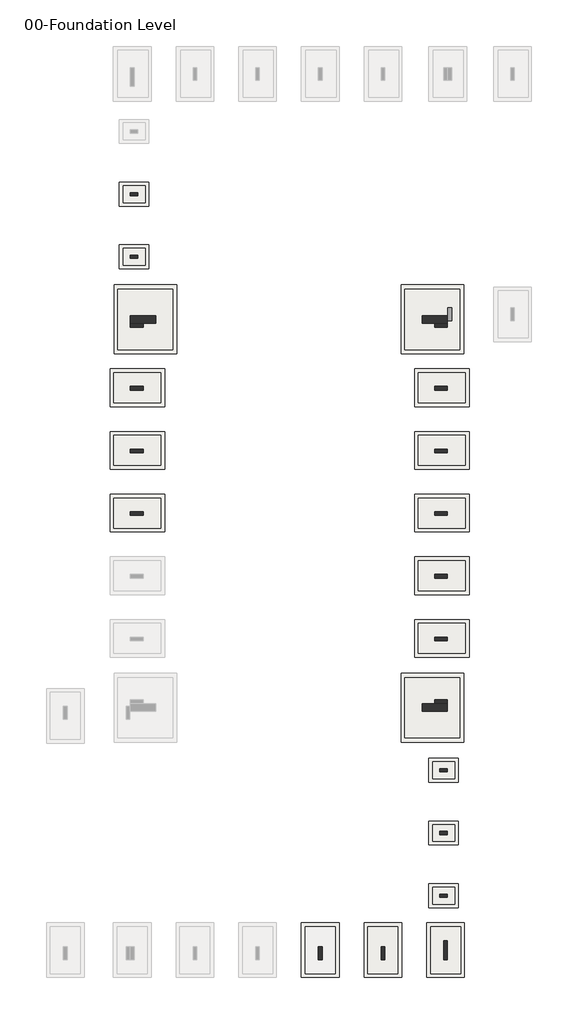
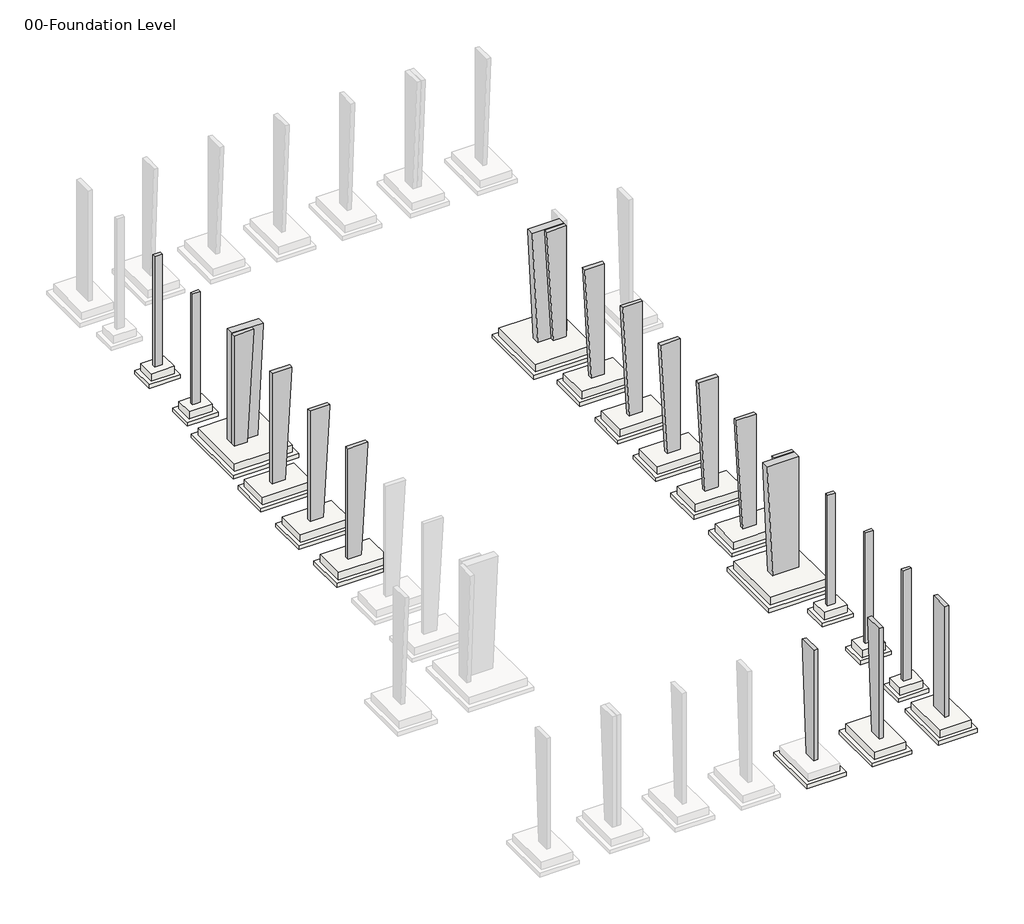
# One storey, part 2 of 4: 37 slabs, 22 columns.
"""IFC4 building model written with IfcOpenShell, lengths in millimetres."""

from ifc_helpers import new_model, si_unit, frame, origin, place, context, project, spatial, polyline, outline, extrude, faceted_brep, element, save

model = new_model("IFC4")

# Units and contexts
model_context = context("Model", 3, world=origin())
ifc_project = project(units=[si_unit("LENGTHUNIT", "METRE", prefix="MILLI")], contexts=[model_context])

# Site, building, storey
site = spatial("IfcSite", under=ifc_project)
building = spatial("IfcBuilding", under=site)
storey = spatial("IfcBuildingStorey", under=building, Name="00-Foundation Level", Elevation=-2000.0)

# Columns
placement = place(None, origin())
element("IfcColumn", 1, ObjectType="Frame Col.2 : 1500x300", at=placement, inside=storey, context=model_context, shape_type="Brep", body=[
    faceted_brep([(49483.2245514, 20339.9999998, -1100.0), (50483.2245514, 20339.9999998, -1100.0), (50483.2245514, 20339.9999998, 7800.0), (48983.2245514, 20339.9999998, 7800.0), (48989.9661245, 20339.9999998, 7680.0), (48983.2245514, 20639.9999998, 7800.0), (48989.9661245, 20639.9999998, 7680.0), (49483.2245514, 20639.9999998, -1100.0), (50483.2245514, 20639.9999998, -1100.0), (50483.2245514, 20639.9999998, 7800.0), (50483.2245514, 20639.9999998, 7680.0)], [[[0, 1, 2, 3, 4]], [[0, 4, 3, 5, 6, 7]], [[8, 7, 6, 5, 9, 10]], [[2, 1, 8, 10, 9]], [[1, 0, 7, 8]], [[3, 2, 9, 5]]]),
])
element("IfcColumn", 2, ObjectType="Frame Col.2 : 1500x300", at=placement, inside=storey, context=model_context, shape_type="Brep", body=[
    faceted_brep([(40183.2245515, 899.7448196, -1100.0), (40183.2245515, -100.2551804, -1100.0), (40183.2245515, -100.2551804, 7680.0), (40183.2245515, -100.2551804, 7800.0), (40183.2245515, 1399.7448196, 7800.0), (40183.2245515, 1393.0032466, 7680.0), (40483.2245515, 1399.7448196, 7800.0), (40483.2245515, 1393.0032466, 7680.0), (40483.2245515, 899.7448196, -1100.0), (40483.2245515, -100.2551804, -1100.0), (40483.2245515, -100.2551804, 7800.0), (40483.2245515, -100.2551804, 7680.0)], [[[0, 1, 2, 3, 4, 5]], [[0, 5, 4, 6, 7, 8]], [[9, 8, 7, 6, 10, 11]], [[3, 2, 1, 9, 11, 10]], [[1, 0, 8, 9]], [[4, 3, 10, 6]]]),
])
element("IfcColumn", 3, ObjectType="Frame Col.2 : 1500x300", at=placement, inside=storey, context=model_context, shape_type="Brep", body=[
    faceted_brep([(45183.2245515, 899.7448196, -1100.0), (45183.2245515, -100.2551804, -1100.0), (45183.2245515, -100.2551804, 7680.0), (45183.2245515, -100.2551804, 7800.0), (45183.2245515, 1399.7448196, 7800.0), (45183.2245515, 1393.0032466, 7680.0), (45483.2245515, 1399.7448196, 7800.0), (45483.2245515, 1393.0032466, 7680.0), (45483.2245515, 899.7448196, -1100.0), (45483.2245515, -100.2551804, -1100.0), (45483.2245515, -100.2551804, 7800.0), (45483.2245515, -100.2551804, 7680.0)], [[[0, 1, 2, 3, 4, 5]], [[0, 5, 4, 6, 7, 8]], [[9, 8, 7, 6, 10, 11]], [[3, 2, 1, 9, 11, 10]], [[1, 0, 8, 9]], [[4, 3, 10, 6]]]),
])
element("IfcColumn", 4, ObjectType="Frame Col.2 : 1500x300", at=placement, inside=storey, context=model_context, shape_type="Brep", body=[
    faceted_brep([(49483.2245514, 25339.9999988, -1100.0), (50483.2245514, 25339.9999988, -1100.0), (50483.2245514, 25339.9999988, 7680.0), (50483.2245514, 25339.9999988, 7800.0), (48983.2245514, 25339.9999988, 7800.0), (48989.9661245, 25339.9999988, 7680.0), (49067.4942144, 25339.9999988, 6300.0), (48983.2245514, 25639.9999988, 7800.0), (48989.9661245, 25639.9999988, 7680.0), (49067.4942144, 25639.9999988, 6300.0), (49483.2245514, 25639.9999988, -1100.0), (50483.2245514, 25639.9999988, -1100.0), (50483.2245514, 25639.9999988, 7800.0), (50483.2245514, 25639.9999988, 7680.0)], [[[0, 1, 2, 3, 4, 5, 6]], [[0, 6, 5, 4, 7, 8, 9, 10]], [[11, 10, 9, 8, 7, 12, 13]], [[3, 2, 1, 11, 13, 12]], [[1, 0, 10, 11]], [[4, 3, 12, 7]]]),
])
element("IfcColumn", 5, ObjectType="Frame Col.2 : 1500x300", at=placement, inside=storey, context=model_context, shape_type="Brep", body=[
    faceted_brep([(49483.2245514, 30339.9999988, -1100.0), (50483.2245514, 30339.9999988, -1100.0), (50483.2245514, 30339.9999988, 7680.0), (50483.2245514, 30339.9999988, 7800.0), (48983.2245514, 30339.9999988, 7800.0), (48989.9661245, 30339.9999988, 7680.0), (49067.4942144, 30339.9999988, 6300.0), (48983.2245514, 30639.9999988, 7800.0), (48989.9661245, 30639.9999988, 7680.0), (49067.4942144, 30639.9999988, 6300.0), (49483.2245514, 30639.9999988, -1100.0), (50483.2245514, 30639.9999988, -1100.0), (50483.2245514, 30639.9999988, 7800.0), (50483.2245514, 30639.9999988, 7680.0)], [[[0, 1, 2, 3, 4, 5, 6]], [[0, 6, 5, 4, 7, 8, 9, 10]], [[11, 10, 9, 8, 7, 12, 13]], [[3, 2, 1, 11, 13, 12]], [[1, 0, 10, 11]], [[4, 3, 12, 7]]]),
])
element("IfcColumn", 6, ObjectType="Frame Col.2 : 1500x300", at=placement, inside=storey, context=model_context, shape_type="Brep", body=[
    faceted_brep([(49483.2245514, 35339.9999988, -1100.0), (50483.2245514, 35339.9999988, -1100.0), (50483.2245514, 35339.9999988, 7680.0), (50483.2245514, 35339.9999988, 7800.0), (48983.2245514, 35339.9999988, 7800.0), (48989.9661245, 35339.9999988, 7680.0), (49067.4942144, 35339.9999988, 6300.0), (48983.2245514, 35639.9999988, 7800.0), (48989.9661245, 35639.9999988, 7680.0), (49067.4942144, 35639.9999988, 6300.0), (49483.2245514, 35639.9999988, -1100.0), (50483.2245514, 35639.9999988, -1100.0), (50483.2245514, 35639.9999988, 7800.0), (50483.2245514, 35639.9999988, 7680.0)], [[[0, 1, 2, 3, 4, 5, 6]], [[0, 6, 5, 4, 7, 8, 9, 10]], [[11, 10, 9, 8, 7, 12, 13]], [[3, 2, 1, 11, 13, 12]], [[1, 0, 10, 11]], [[4, 3, 12, 7]]]),
])
element("IfcColumn", 7, ObjectType="Frame Col.2 : 1500x300", at=placement, inside=storey, context=model_context, shape_type="Brep", body=[
    faceted_brep([(26183.2245516, 35639.9999988, -1100.0), (25183.2245516, 35639.9999988, -1100.0), (25183.2245516, 35639.9999988, 7680.0), (25183.2245516, 35639.9999988, 7800.0), (26683.2245516, 35639.9999988, 7800.0), (26676.4829785, 35639.9999988, 7680.0), (26598.9548887, 35639.9999988, 6300.0), (26683.2245516, 35339.9999988, 7800.0), (26676.4829785, 35339.9999988, 7680.0), (26598.9548887, 35339.9999988, 6300.0), (26183.2245516, 35339.9999988, -1100.0), (25183.2245516, 35339.9999988, -1100.0), (25183.2245516, 35339.9999988, 7800.0), (25183.2245516, 35339.9999988, 7680.0)], [[[0, 1, 2, 3, 4, 5, 6]], [[0, 6, 5, 4, 7, 8, 9, 10]], [[11, 10, 9, 8, 7, 12, 13]], [[3, 2, 1, 11, 13, 12]], [[1, 0, 10, 11]], [[4, 3, 12, 7]]]),
])
element("IfcColumn", 8, ObjectType="Frame Col.2 : 1500x300", at=placement, inside=storey, context=model_context, shape_type="Brep", body=[
    faceted_brep([(49483.2245514, 40339.9999988, -1100.0), (50483.2245514, 40339.9999988, -1100.0), (50483.2245514, 40339.9999988, 7680.0), (50483.2245514, 40339.9999988, 7800.0), (48983.2245514, 40339.9999988, 7800.0), (48989.9661245, 40339.9999988, 7680.0), (49067.4942144, 40339.9999988, 6300.0), (48983.2245514, 40639.9999988, 7800.0), (48989.9661245, 40639.9999988, 7680.0), (49067.4942144, 40639.9999988, 6300.0), (49483.2245514, 40639.9999988, -1100.0), (50483.2245514, 40639.9999988, -1100.0), (50483.2245514, 40639.9999988, 7800.0), (50483.2245514, 40639.9999988, 7680.0)], [[[0, 1, 2, 3, 4, 5, 6]], [[0, 6, 5, 4, 7, 8, 9, 10]], [[11, 10, 9, 8, 7, 12, 13]], [[3, 2, 1, 11, 13, 12]], [[1, 0, 10, 11]], [[4, 3, 12, 7]]]),
])
element("IfcColumn", 9, ObjectType="Frame Col.2 : 1500x300", at=placement, inside=storey, context=model_context, shape_type="Brep", body=[
    faceted_brep([(26183.2245516, 40639.9999988, -1100.0), (25183.2245516, 40639.9999988, -1100.0), (25183.2245516, 40639.9999988, 7680.0), (25183.2245516, 40639.9999988, 7800.0), (26683.2245516, 40639.9999988, 7800.0), (26676.4829785, 40639.9999988, 7680.0), (26598.9548887, 40639.9999988, 6300.0), (26683.2245516, 40339.9999988, 7800.0), (26676.4829785, 40339.9999988, 7680.0), (26598.9548887, 40339.9999988, 6300.0), (26183.2245516, 40339.9999988, -1100.0), (25183.2245516, 40339.9999988, -1100.0), (25183.2245516, 40339.9999988, 7800.0), (25183.2245516, 40339.9999988, 7680.0)], [[[0, 1, 2, 3, 4, 5, 6]], [[0, 6, 5, 4, 7, 8, 9, 10]], [[11, 10, 9, 8, 7, 12, 13]], [[3, 2, 1, 11, 13, 12]], [[1, 0, 10, 11]], [[4, 3, 12, 7]]]),
])
element("IfcColumn", 10, ObjectType="Frame Col.2 : 1500x300", at=placement, inside=storey, context=model_context, shape_type="Brep", body=[
    faceted_brep([(49483.2245514, 45339.9999993, -1100.0), (50483.2245514, 45339.9999993, -1100.0), (50483.2245514, 45339.9999993, 7680.0), (50483.2245514, 45339.9999993, 7800.0), (48983.2245514, 45339.9999993, 7800.0), (48989.9661245, 45339.9999993, 7680.0), (49067.4942144, 45339.9999993, 6300.0), (48983.2245514, 45639.9999993, 7800.0), (48989.9661245, 45639.9999993, 7680.0), (49067.4942144, 45639.9999993, 6300.0), (49483.2245514, 45639.9999993, -1100.0), (50483.2245514, 45639.9999993, -1100.0), (50483.2245514, 45639.9999993, 7800.0), (50483.2245514, 45639.9999993, 7680.0)], [[[0, 1, 2, 3, 4, 5, 6]], [[0, 6, 5, 4, 7, 8, 9, 10]], [[11, 10, 9, 8, 7, 12, 13]], [[3, 2, 1, 11, 13, 12]], [[1, 0, 10, 11]], [[4, 3, 12, 7]]]),
])
element("IfcColumn", 11, ObjectType="Frame Col.2 : 1500x300", at=placement, inside=storey, context=model_context, shape_type="Brep", body=[
    faceted_brep([(26183.2245516, 45639.9999993, -1100.0), (25183.2245516, 45639.9999993, -1100.0), (25183.2245516, 45639.9999993, 7680.0), (25183.2245516, 45639.9999993, 7800.0), (26683.2245516, 45639.9999993, 7800.0), (26676.4829785, 45639.9999993, 7680.0), (26598.9548887, 45639.9999993, 6300.0), (26683.2245516, 45339.9999993, 7800.0), (26676.4829785, 45339.9999993, 7680.0), (26598.9548887, 45339.9999993, 6300.0), (26183.2245516, 45339.9999993, -1100.0), (25183.2245516, 45339.9999993, -1100.0), (25183.2245516, 45339.9999993, 7800.0), (25183.2245516, 45339.9999993, 7680.0)], [[[0, 1, 2, 3, 4, 5, 6]], [[0, 6, 5, 4, 7, 8, 9, 10]], [[11, 10, 9, 8, 7, 12, 13]], [[3, 2, 1, 11, 13, 12]], [[1, 0, 10, 11]], [[4, 3, 12, 7]]]),
])
element("IfcColumn", 12, ObjectType="Frame Col.2 : 1500x300", at=placement, inside=storey, context=model_context, shape_type="Brep", body=[
    faceted_brep([(49483.2245514, 50339.9999991, -1100.0), (50483.2245514, 50339.9999991, -1100.0), (50483.2245514, 50339.9999991, 7680.0), (50483.2245514, 50339.9999991, 7800.0), (48983.2245514, 50339.9999991, 7800.0), (48989.9661245, 50339.9999991, 7680.0), (48983.2245514, 50639.9999991, 7800.0), (48989.9661245, 50639.9999991, 7680.0), (49483.2245514, 50639.9999991, -1100.0), (50483.2245514, 50639.9999991, -1100.0), (50483.2245514, 50639.9999991, 7800.0)], [[[0, 1, 2, 3, 4, 5]], [[0, 5, 4, 6, 7, 8]], [[9, 8, 7, 6, 10]], [[3, 2, 1, 9, 10]], [[1, 0, 8, 9]], [[4, 3, 10, 6]]]),
])
element("IfcColumn", 13, ObjectType="Frame Col.2 : 1500x300", at=placement, inside=storey, context=model_context, shape_type="Brep", body=[
    faceted_brep([(26183.2245516, 50639.9999991, -1100.0), (25183.2245516, 50639.9999991, -1100.0), (25183.2245516, 50639.9999991, 7800.0), (26683.2245516, 50639.9999991, 7800.0), (26676.4829785, 50639.9999991, 7680.0), (26683.2245516, 50339.9999991, 7800.0), (26676.4829785, 50339.9999991, 7680.0), (26183.2245516, 50339.9999991, -1100.0), (25183.2245516, 50339.9999991, -1100.0), (25183.2245516, 50339.9999991, 7800.0), (25183.2245516, 50339.9999991, 7680.0)], [[[0, 1, 2, 3, 4]], [[0, 4, 3, 5, 6, 7]], [[8, 7, 6, 5, 9, 10]], [[2, 1, 8, 10, 9]], [[1, 0, 7, 8]], [[3, 2, 9, 5]]]),
])
element("IfcColumn", 14, ObjectType="Frame Col.2 : 2400x600", at=placement, inside=storey, context=model_context, shape_type="Brep", body=[
    faceted_brep([(48483.2245514, 50679.9999988, -1100.0), (50483.2245514, 50679.9999988, -1100.0), (50483.2245514, 50679.9999988, 7800.0), (48083.2245514, 50679.9999988, 7800.0), (48088.6178099, 50679.9999988, 7680.0), (48083.2245514, 51279.9999988, 7800.0), (48088.6178099, 51279.9999988, 7680.0), (48483.2245514, 51279.9999988, -1100.0), (50483.2245514, 51279.9999988, -1100.0), (50483.2245514, 51279.9999988, 7800.0), (50483.2245514, 51279.9999988, 7680.0)], [[[0, 1, 2, 3, 4]], [[0, 4, 3, 5, 6, 7]], [[8, 7, 6, 5, 9, 10]], [[2, 1, 8, 10, 9]], [[1, 0, 7, 8]], [[3, 2, 9, 5]]]),
])
element("IfcColumn", 15, ObjectType="Frame Col.2 : 2400x600", at=placement, inside=storey, context=model_context, shape_type="Brep", body=[
    faceted_brep([(27183.2245516, 51279.9999991, -1100.0), (25183.2245516, 51279.9999991, -1100.0), (25183.2245516, 51279.9999991, 7680.0), (25183.2245516, 51279.9999991, 7800.0), (27583.2245516, 51279.9999991, 7800.0), (27577.8312932, 51279.9999991, 7680.0), (27583.2245516, 50679.9999991, 7800.0), (27577.8312932, 50679.9999991, 7680.0), (27183.2245516, 50679.9999991, -1100.0), (25183.2245516, 50679.9999991, -1100.0), (25183.2245516, 50679.9999991, 7800.0)], [[[0, 1, 2, 3, 4, 5]], [[0, 5, 4, 6, 7, 8]], [[9, 8, 7, 6, 10]], [[3, 2, 1, 9, 10]], [[1, 0, 8, 9]], [[4, 3, 10, 6]]]),
])
element("IfcColumn", 16, ObjectType="Frame Col.2 : 2400x600", at=placement, inside=storey, context=model_context, shape_type="Brep", body=[
    faceted_brep([(48483.2245514, 19699.9999993, -1100.0), (50483.2245514, 19699.9999993, -1100.0), (50483.2245514, 19699.9999993, 7680.0), (50483.2245514, 19699.9999993, 7800.0), (48083.2245514, 19699.9999993, 7800.0), (48088.6178099, 19699.9999993, 7680.0), (48083.2245514, 20299.9999993, 7800.0), (48088.6178099, 20299.9999993, 7680.0), (48483.2245514, 20299.9999993, -1100.0), (50483.2245514, 20299.9999993, -1100.0), (50483.2245514, 20299.9999993, 7800.0)], [[[0, 1, 2, 3, 4, 5]], [[0, 5, 4, 6, 7, 8]], [[9, 8, 7, 6, 10]], [[3, 2, 1, 9, 10]], [[1, 0, 8, 9]], [[4, 3, 10, 6]]]),
])
element("IfcColumn", 17, ObjectType="M_Concrete-Rectangular-Column : 250 x 600mm", at=placement, inside=storey, context=model_context, shape_type="Brep", body=[
    faceted_brep([(25183.2245516, 61104.74482, -1100.0), (25783.2245516, 61104.74482, -1100.0), (25783.2245516, 60854.74482, -1100.0), (25183.2245516, 60854.74482, -1100.0), (25183.2245516, 61104.74482, 7680.0), (25183.2245516, 61104.74482, 7800.0), (25783.2245516, 61104.74482, 7800.0), (25783.2245516, 61104.74482, 7680.0), (25183.2245516, 60854.74482, 7680.0), (25183.2245516, 60854.74482, 7800.0), (25783.2245516, 60854.74482, 7680.0), (25783.2245516, 60854.74482, 7800.0)], [[[0, 1, 2, 3]], [[1, 0, 4, 5, 6, 7]], [[0, 3, 8, 9, 5, 4]], [[3, 2, 10, 11, 9, 8]], [[2, 1, 7, 6, 11, 10]], [[6, 5, 9, 11]]]),
])
element("IfcColumn", 18, ObjectType="M_Concrete-Rectangular-Column : 250 x 600mm", at=placement, inside=storey, context=model_context, shape_type="Brep", body=[
    faceted_brep([(25183.2245516, 56104.9999988, -1100.0), (25783.2245516, 56104.9999988, -1100.0), (25783.2245516, 55854.9999988, -1100.0), (25183.2245516, 55854.9999988, -1100.0), (25183.2245516, 56104.9999988, 7680.0), (25183.2245516, 56104.9999988, 7800.0), (25783.2245516, 56104.9999988, 7800.0), (25783.2245516, 56104.9999988, 7680.0), (25183.2245516, 55854.9999988, 7680.0), (25183.2245516, 55854.9999988, 7800.0), (25783.2245516, 55854.9999988, 7680.0), (25783.2245516, 55854.9999988, 7800.0)], [[[0, 1, 2, 3]], [[1, 0, 4, 5, 6, 7]], [[0, 3, 8, 9, 5, 4]], [[3, 2, 10, 11, 9, 8]], [[2, 1, 7, 6, 11, 10]], [[6, 5, 9, 11]]]),
])
element("IfcColumn", 19, ObjectType="M_Concrete-Rectangular-Column : 250 x 600mm", at=placement, inside=storey, context=model_context, shape_type="Brep", body=[
    faceted_brep([(50483.2245514, 4874.9999995, -1100.0), (49883.2245514, 4874.9999995, -1100.0), (49883.2245514, 5124.9999995, -1100.0), (50483.2245514, 5124.9999995, -1100.0), (50483.2245514, 4874.9999995, 7680.0), (50483.2245514, 4874.9999995, 7800.0), (49883.2245514, 4874.9999995, 7800.0), (49883.2245514, 4874.9999995, 7680.0), (50483.2245514, 5124.9999995, 7680.0), (50483.2245514, 5124.9999995, 7800.0), (49883.2245514, 5124.9999995, 7680.0), (49883.2245514, 5124.9999995, 7800.0)], [[[0, 1, 2, 3]], [[1, 0, 4, 5, 6, 7]], [[0, 3, 8, 9, 5, 4]], [[3, 2, 10, 11, 9, 8]], [[2, 1, 7, 6, 11, 10]], [[6, 5, 9, 11]]]),
])
element("IfcColumn", 20, ObjectType="M_Concrete-Rectangular-Column : 250 x 600mm", at=placement, inside=storey, context=model_context, shape_type="Brep", body=[
    faceted_brep([(50483.2245514, 9874.7448207, -1100.0), (49883.2245514, 9874.7448207, -1100.0), (49883.2245514, 10124.7448207, -1100.0), (50483.2245514, 10124.7448207, -1100.0), (50483.2245514, 9874.7448207, 7680.0), (50483.2245514, 9874.7448207, 7800.0), (49883.2245514, 9874.7448207, 7800.0), (49883.2245514, 9874.7448207, 7680.0), (50483.2245514, 10124.7448207, 7680.0), (50483.2245514, 10124.7448207, 7800.0), (50483.2245514, 9874.9999995, 7800.0), (49883.2245514, 10124.7448207, 7680.0), (49883.2245514, 10124.7448207, 7800.0), (49883.2245514, 9874.9999995, 7800.0)], [[[0, 1, 2, 3]], [[1, 0, 4, 5, 6, 7]], [[0, 3, 8, 9, 10, 5, 4]], [[3, 2, 11, 12, 9, 8]], [[2, 1, 7, 6, 13, 12, 11]], [[6, 5, 10, 9, 12, 13]]]),
])
element("IfcColumn", 21, ObjectType="M_Concrete-Rectangular-Column : 250 x 600mm", at=placement, inside=storey, context=model_context, shape_type="Brep", body=[
    faceted_brep([(50483.2245514, 14874.9999995, -1100.0), (49883.2245514, 14874.9999995, -1100.0), (49883.2245514, 15124.9999995, -1100.0), (50483.2245514, 15124.9999995, -1100.0), (50483.2245514, 14874.9999995, 7680.0), (50483.2245514, 14874.9999995, 7800.0), (49883.2245514, 14874.9999995, 7800.0), (49883.2245514, 14874.9999995, 7680.0), (50483.2245514, 15124.9999995, 7680.0), (50483.2245514, 15124.9999995, 7800.0), (49883.2245514, 15124.9999995, 7680.0), (49883.2245514, 15124.9999995, 7800.0)], [[[0, 1, 2, 3]], [[1, 0, 4, 5, 6, 7]], [[0, 3, 8, 9, 5, 4]], [[3, 2, 10, 11, 9, 8]], [[2, 1, 7, 6, 11, 10]], [[6, 5, 9, 11]]]),
])
element("IfcColumn", 22, ObjectType="M_Concrete-Rectangular-Column : 300 x 1500mm", at=placement, inside=storey, context=model_context, shape_type="Brep", body=[
    faceted_brep([(50483.2245514, 1399.7448196, -1100.0), (50483.2245514, -100.2551804, -1100.0), (50183.2245514, -100.2551804, -1100.0), (50183.2245514, 1399.7448196, -1100.0), (50483.2245514, 1399.7448196, 7680.0), (50483.2245514, 1399.7448196, 7800.0), (50483.2245514, -100.2551804, 7800.0), (50183.2245514, 1399.7448196, 7680.0), (50183.2245514, 1399.7448196, 7800.0), (50183.2245514, -100.2551804, 7680.0), (50183.2245514, -100.2551804, 7800.0)], [[[0, 1, 2, 3]], [[1, 0, 4, 5, 6]], [[0, 3, 7, 8, 5, 4]], [[3, 2, 9, 10, 8, 7]], [[2, 1, 6, 10, 9]], [[6, 5, 8, 10]]]),
])

# Slabs
element("IfcSlab", 23, ObjectType="M_Footing-Rectangular : PC 2-2350 x 1900 x 300mm", at=placement, inside=storey, context=model_context, shape_type="SweptSolid", body=[
    extrude(outline(polyline([(26658.2245516, 61929.9999988), (26658.2245516, 60029.9999988), (24308.2245516, 60029.9999988), (24308.2245516, 61929.9999988), (26658.2245516, 61929.9999988)])), frame((0.0, 0.0, -2000.0), z_axis=(0.0, 0.0, 1.0), x_axis=(1.0, 0.0, 0.0)), (0.0, 0.0, 1.0), 300.0),
])
element("IfcSlab", 24, ObjectType="M_Footing-Rectangular : PC 2-2350 x 1900 x 300mm", at=placement, inside=storey, context=model_context, shape_type="SweptSolid", body=[
    extrude(outline(polyline([(26658.2245516, 56929.9999988), (26658.2245516, 55029.9999988), (24308.2245516, 55029.9999988), (24308.2245516, 56929.9999988), (26658.2245516, 56929.9999988)])), frame((0.0, 0.0, -2000.0), z_axis=(0.0, 0.0, 1.0), x_axis=(1.0, 0.0, 0.0)), (0.0, 0.0, 1.0), 300.0),
])
element("IfcSlab", 25, ObjectType="M_Footing-Rectangular : PC 2-2350 x 1900 x 300mm", at=placement, inside=storey, context=model_context, shape_type="SweptSolid", body=[
    extrude(outline(polyline([(51358.2245514, 15949.9999995), (51358.2245514, 14049.9999995), (49008.2245514, 14049.9999995), (49008.2245514, 15949.9999995), (51358.2245514, 15949.9999995)])), frame((0.0, 0.0, -2000.0), z_axis=(0.0, 0.0, 1.0), x_axis=(1.0, 0.0, 0.0)), (0.0, 0.0, 1.0), 300.0),
])
element("IfcSlab", 26, ObjectType="M_Footing-Rectangular : PC 2-2350 x 1900 x 300mm", at=placement, inside=storey, context=model_context, shape_type="SweptSolid", body=[
    extrude(outline(polyline([(51358.2245514, 10949.9999995), (51358.2245514, 9049.9999995), (49008.2245514, 9049.9999995), (49008.2245514, 10949.9999995), (51358.2245514, 10949.9999995)])), frame((0.0, 0.0, -2000.0), z_axis=(0.0, 0.0, 1.0), x_axis=(1.0, 0.0, 0.0)), (0.0, 0.0, 1.0), 300.0),
])
element("IfcSlab", 27, ObjectType="M_Footing-Rectangular : PC 2-2350 x 1900 x 300mm", at=placement, inside=storey, context=model_context, shape_type="SweptSolid", body=[
    extrude(outline(polyline([(51358.2245514, 5949.9999995), (51358.2245514, 4049.9999995), (49008.2245514, 4049.9999995), (49008.2245514, 5949.9999995), (51358.2245514, 5949.9999995)])), frame((0.0, 0.0, -2000.0), z_axis=(0.0, 0.0, 1.0), x_axis=(1.0, 0.0, 0.0)), (0.0, 0.0, 1.0), 300.0),
])
element("IfcSlab", 28, ObjectType="M_Footing-Rectangular : PC 3-5500 x 5000 x 300mm", at=placement, inside=storey, context=model_context, shape_type="SweptSolid", body=[
    extrude(outline(polyline([(46783.2245514, 53729.9999991), (51783.2245514, 53729.9999991), (51783.2245514, 48229.9999991), (46783.2245514, 48229.9999991), (46783.2245514, 53729.9999991)])), frame((0.0, 0.0, -2000.0), z_axis=(0.0, 0.0, 1.0), x_axis=(1.0, 0.0, 0.0)), (0.0, 0.0, 1.0), 300.0),
])
element("IfcSlab", 29, ObjectType="M_Footing-Rectangular : PC 3-5500 x 5000 x 300mm", at=placement, inside=storey, context=model_context, shape_type="SweptSolid", body=[
    extrude(outline(polyline([(23883.2245516, 53729.9999991), (28883.2245516, 53729.9999991), (28883.2245516, 48229.9999991), (23883.2245516, 48229.9999991), (23883.2245516, 53729.9999991)])), frame((0.0, 0.0, -2000.0), z_axis=(0.0, 0.0, 1.0), x_axis=(1.0, 0.0, 0.0)), (0.0, 0.0, 1.0), 300.0),
])
element("IfcSlab", 30, ObjectType="M_Footing-Rectangular : PC 3-5500 x 5000 x 300mm", at=placement, inside=storey, context=model_context, shape_type="SweptSolid", body=[
    extrude(outline(polyline([(46783.2245514, 22749.9999993), (51783.2245514, 22749.9999993), (51783.2245514, 17249.9999993), (46783.2245514, 17249.9999993), (46783.2245514, 22749.9999993)])), frame((0.0, 0.0, -2000.0), z_axis=(0.0, 0.0, 1.0), x_axis=(1.0, 0.0, 0.0)), (0.0, 0.0, 1.0), 300.0),
])
element("IfcSlab", 31, ObjectType="M_Footing-Rectangular : PC-4350 x 3000 x 300mm", at=placement, inside=storey, context=model_context, shape_type="SweptSolid", body=[
    extrude(outline(polyline([(51833.2245514, 2825.0), (51833.2245514, -1525.0), (48833.2245514, -1525.0), (48833.2245514, 2825.0), (51833.2245514, 2825.0)])), frame((0.0, 0.0, -2000.0), z_axis=(0.0, 0.0, 1.0), x_axis=(1.0, 0.0, 0.0)), (0.0, 0.0, 1.0), 300.0),
])
element("IfcSlab", 32, ObjectType="M_Footing-Rectangular : PC-4350 x 3000 x 300mm", at=placement, inside=storey, context=model_context, shape_type="SweptSolid", body=[
    extrude(outline(polyline([(46833.2245515, 2825.0), (46833.2245515, -1525.0), (43833.2245515, -1525.0), (43833.2245515, 2825.0), (46833.2245515, 2825.0)])), frame((0.0, 0.0, -2000.0), z_axis=(0.0, 0.0, 1.0), x_axis=(1.0, 0.0, 0.0)), (0.0, 0.0, 1.0), 300.0),
])
element("IfcSlab", 33, ObjectType="M_Footing-Rectangular : PC-4350 x 3000 x 300mm", at=placement, inside=storey, context=model_context, shape_type="SweptSolid", body=[
    extrude(outline(polyline([(41833.2245515, 2825.0), (41833.2245515, -1525.0), (38833.2245515, -1525.0), (38833.2245515, 2825.0), (41833.2245515, 2825.0)])), frame((0.0, 0.0, -2000.0), z_axis=(0.0, 0.0, 1.0), x_axis=(1.0, 0.0, 0.0)), (0.0, 0.0, 1.0), 300.0),
])
element("IfcSlab", 34, ObjectType="M_Footing-Rectangular : PC-4350 x 3000 x 300mm", at=placement, inside=storey, context=model_context, shape_type="SweptSolid", body=[
    extrude(outline(polyline([(23564.9999997, 47029.7448203), (27914.9999997, 47029.7448203), (27914.9999997, 44029.7448203), (23564.9999997, 44029.7448203), (23564.9999997, 47029.7448203)])), frame((0.0, 0.0, -2000.0), z_axis=(0.0, 0.0, 1.0), x_axis=(1.0, 0.0, 0.0)), (0.0, 0.0, 1.0), 300.0),
])
element("IfcSlab", 35, ObjectType="M_Footing-Rectangular : PC-4350 x 3000 x 300mm", at=placement, inside=storey, context=model_context, shape_type="SweptSolid", body=[
    extrude(outline(polyline([(47864.9999995, 47029.7448203), (52214.9999995, 47029.7448203), (52214.9999995, 44029.7448203), (47864.9999995, 44029.7448203), (47864.9999995, 47029.7448203)])), frame((0.0, 0.0, -2000.0), z_axis=(0.0, 0.0, 1.0), x_axis=(1.0, 0.0, 0.0)), (0.0, 0.0, 1.0), 300.0),
])
element("IfcSlab", 36, ObjectType="M_Footing-Rectangular : PC-4350 x 3000 x 300mm", at=placement, inside=storey, context=model_context, shape_type="SweptSolid", body=[
    extrude(outline(polyline([(23564.9999997, 42029.7448203), (27914.9999997, 42029.7448203), (27914.9999997, 39029.7448203), (23564.9999997, 39029.7448203), (23564.9999997, 42029.7448203)])), frame((0.0, 0.0, -2000.0), z_axis=(0.0, 0.0, 1.0), x_axis=(1.0, 0.0, 0.0)), (0.0, 0.0, 1.0), 300.0),
])
element("IfcSlab", 37, ObjectType="M_Footing-Rectangular : PC-4350 x 3000 x 300mm", at=placement, inside=storey, context=model_context, shape_type="SweptSolid", body=[
    extrude(outline(polyline([(47864.9999995, 42029.7448203), (52214.9999995, 42029.7448203), (52214.9999995, 39029.7448203), (47864.9999995, 39029.7448203), (47864.9999995, 42029.7448203)])), frame((0.0, 0.0, -2000.0), z_axis=(0.0, 0.0, 1.0), x_axis=(1.0, 0.0, 0.0)), (0.0, 0.0, 1.0), 300.0),
])
element("IfcSlab", 38, ObjectType="M_Footing-Rectangular : PC-4350 x 3000 x 300mm", at=placement, inside=storey, context=model_context, shape_type="SweptSolid", body=[
    extrude(outline(polyline([(23564.9999997, 37029.7448203), (27914.9999997, 37029.7448203), (27914.9999997, 34029.7448203), (23564.9999997, 34029.7448203), (23564.9999997, 37029.7448203)])), frame((0.0, 0.0, -2000.0), z_axis=(0.0, 0.0, 1.0), x_axis=(1.0, 0.0, 0.0)), (0.0, 0.0, 1.0), 300.0),
])
element("IfcSlab", 39, ObjectType="M_Footing-Rectangular : PC-4350 x 3000 x 300mm", at=placement, inside=storey, context=model_context, shape_type="SweptSolid", body=[
    extrude(outline(polyline([(47864.9999995, 37029.7448203), (52214.9999995, 37029.7448203), (52214.9999995, 34029.7448203), (47864.9999995, 34029.7448203), (47864.9999995, 37029.7448203)])), frame((0.0, 0.0, -2000.0), z_axis=(0.0, 0.0, 1.0), x_axis=(1.0, 0.0, 0.0)), (0.0, 0.0, 1.0), 300.0),
])
element("IfcSlab", 40, ObjectType="M_Footing-Rectangular : PC-4350 x 3000 x 300mm", at=placement, inside=storey, context=model_context, shape_type="SweptSolid", body=[
    extrude(outline(polyline([(47864.9999995, 32029.7448203), (52214.9999995, 32029.7448203), (52214.9999995, 29029.7448203), (47864.9999995, 29029.7448203), (47864.9999995, 32029.7448203)])), frame((0.0, 0.0, -2000.0), z_axis=(0.0, 0.0, 1.0), x_axis=(1.0, 0.0, 0.0)), (0.0, 0.0, 1.0), 300.0),
])
element("IfcSlab", 41, ObjectType="M_Footing-Rectangular : PC-4350 x 3000 x 300mm", at=placement, inside=storey, context=model_context, shape_type="SweptSolid", body=[
    extrude(outline(polyline([(47864.9999995, 27029.7448203), (52214.9999995, 27029.7448203), (52214.9999995, 24029.7448203), (47864.9999995, 24029.7448203), (47864.9999995, 27029.7448203)])), frame((0.0, 0.0, -2000.0), z_axis=(0.0, 0.0, 1.0), x_axis=(1.0, 0.0, 0.0)), (0.0, 0.0, 1.0), 300.0),
])
element("IfcSlab", 42, ObjectType="M_Footing-Rectangular : RC 2-1750 x 1350 x 600mm", at=placement, inside=storey, context=model_context, shape_type="SweptSolid", body=[
    extrude(outline(polyline([(26358.2245516, 61654.9999988), (26358.2245516, 60304.9999988), (24608.2245516, 60304.9999988), (24608.2245516, 61654.9999988), (26358.2245516, 61654.9999988)])), frame((0.0, 0.0, -1700.0), z_axis=(0.0, 0.0, 1.0), x_axis=(1.0, 0.0, 0.0)), (0.0, 0.0, 1.0), 600.0),
])
element("IfcSlab", 43, ObjectType="M_Footing-Rectangular : RC 2-1750 x 1350 x 600mm", at=placement, inside=storey, context=model_context, shape_type="SweptSolid", body=[
    extrude(outline(polyline([(26358.2245516, 56654.9999988), (26358.2245516, 55304.9999988), (24608.2245516, 55304.9999988), (24608.2245516, 56654.9999988), (26358.2245516, 56654.9999988)])), frame((0.0, 0.0, -1700.0), z_axis=(0.0, 0.0, 1.0), x_axis=(1.0, 0.0, 0.0)), (0.0, 0.0, 1.0), 600.0),
])
element("IfcSlab", 44, ObjectType="M_Footing-Rectangular : RC 2-1750 x 1350 x 600mm", at=placement, inside=storey, context=model_context, shape_type="SweptSolid", body=[
    extrude(outline(polyline([(49308.2245514, 14324.9999995), (49308.2245514, 15674.9999995), (51058.2245514, 15674.9999995), (51058.2245514, 14324.9999995), (49308.2245514, 14324.9999995)])), frame((0.0, 0.0, -1700.0), z_axis=(0.0, 0.0, 1.0), x_axis=(1.0, 0.0, 0.0)), (0.0, 0.0, 1.0), 600.0),
])
element("IfcSlab", 45, ObjectType="M_Footing-Rectangular : RC 2-1750 x 1350 x 600mm", at=placement, inside=storey, context=model_context, shape_type="SweptSolid", body=[
    extrude(outline(polyline([(49308.2245514, 9324.9999995), (49308.2245514, 10674.9999995), (51058.2245514, 10674.9999995), (51058.2245514, 9324.9999995), (49308.2245514, 9324.9999995)])), frame((0.0, 0.0, -1700.0), z_axis=(0.0, 0.0, 1.0), x_axis=(1.0, 0.0, 0.0)), (0.0, 0.0, 1.0), 600.0),
])
element("IfcSlab", 46, ObjectType="M_Footing-Rectangular : RC 2-1750 x 1350 x 600mm", at=placement, inside=storey, context=model_context, shape_type="SweptSolid", body=[
    extrude(outline(polyline([(49308.2245514, 4324.9999995), (49308.2245514, 5674.9999995), (51058.2245514, 5674.9999995), (51058.2245514, 4324.9999995), (49308.2245514, 4324.9999995)])), frame((0.0, 0.0, -1700.0), z_axis=(0.0, 0.0, 1.0), x_axis=(1.0, 0.0, 0.0)), (0.0, 0.0, 1.0), 600.0),
])
element("IfcSlab", 47, ObjectType="M_Footing-Rectangular : RC 3- 4800 x 4400 x 600mm 2", at=placement, inside=storey, context=model_context, shape_type="SweptSolid", body=[
    extrude(outline(polyline([(47083.2245514, 53379.9999991), (51483.2245514, 53379.9999991), (51483.2245514, 48579.9999991), (47083.2245514, 48579.9999991), (47083.2245514, 53379.9999991)])), frame((0.0, 0.0, -1700.0), z_axis=(0.0, 0.0, 1.0), x_axis=(1.0, 0.0, 0.0)), (0.0, 0.0, 1.0), 600.0),
])
element("IfcSlab", 48, ObjectType="M_Footing-Rectangular : RC 3- 4800 x 4400 x 600mm 2", at=placement, inside=storey, context=model_context, shape_type="SweptSolid", body=[
    extrude(outline(polyline([(24183.2245516, 53379.9999991), (28583.2245516, 53379.9999991), (28583.2245516, 48579.9999991), (24183.2245516, 48579.9999991), (24183.2245516, 53379.9999991)])), frame((0.0, 0.0, -1700.0), z_axis=(0.0, 0.0, 1.0), x_axis=(1.0, 0.0, 0.0)), (0.0, 0.0, 1.0), 600.0),
])
element("IfcSlab", 49, ObjectType="M_Footing-Rectangular : RC 3- 4800 x 4400 x 600mm 2", at=placement, inside=storey, context=model_context, shape_type="SweptSolid", body=[
    extrude(outline(polyline([(47083.2245514, 22399.9999993), (51483.2245514, 22399.9999993), (51483.2245514, 17599.9999993), (47083.2245514, 17599.9999993), (47083.2245514, 22399.9999993)])), frame((0.0, 0.0, -1700.0), z_axis=(0.0, 0.0, 1.0), x_axis=(1.0, 0.0, 0.0)), (0.0, 0.0, 1.0), 600.0),
])
element("IfcSlab", 50, ObjectType="M_Footing-Rectangular : RC-3750 x 2400 x 600mm", at=placement, inside=storey, context=model_context, shape_type="SweptSolid", body=[
    extrude(outline(polyline([(51533.2245514, 2525.0), (51533.2245514, -1225.0), (49133.2245514, -1225.0), (49133.2245514, 2525.0), (51533.2245514, 2525.0)])), frame((0.0, 0.0, -1700.0), z_axis=(0.0, 0.0, 1.0), x_axis=(1.0, 0.0, 0.0)), (0.0, 0.0, 1.0), 600.0),
])
element("IfcSlab", 51, ObjectType="M_Footing-Rectangular : RC-3750 x 2400 x 600mm", at=placement, inside=storey, context=model_context, shape_type="SweptSolid", body=[
    extrude(outline(polyline([(46533.2245515, 2525.0), (46533.2245515, -1225.0), (44133.2245515, -1225.0), (44133.2245515, 2525.0), (46533.2245515, 2525.0)])), frame((0.0, 0.0, -1700.0), z_axis=(0.0, 0.0, 1.0), x_axis=(1.0, 0.0, 0.0)), (0.0, 0.0, 1.0), 600.0),
])
element("IfcSlab", 52, ObjectType="M_Footing-Rectangular : RC-3750 x 2400 x 600mm", at=placement, inside=storey, context=model_context, shape_type="SweptSolid", body=[
    extrude(outline(polyline([(23864.9999997, 46729.7448203), (27614.9999997, 46729.7448203), (27614.9999997, 44329.7448203), (23864.9999997, 44329.7448203), (23864.9999997, 46729.7448203)])), frame((0.0, 0.0, -1700.0), z_axis=(0.0, 0.0, 1.0), x_axis=(1.0, 0.0, 0.0)), (0.0, 0.0, 1.0), 600.0),
])
element("IfcSlab", 53, ObjectType="M_Footing-Rectangular : RC-3750 x 2400 x 600mm", at=placement, inside=storey, context=model_context, shape_type="SweptSolid", body=[
    extrude(outline(polyline([(51914.9999995, 44329.7448199), (48164.9999995, 44329.7448199), (48164.9999995, 46729.7448199), (51914.9999995, 46729.7448199), (51914.9999995, 44329.7448199)])), frame((0.0, 0.0, -1700.0), z_axis=(0.0, 0.0, 1.0), x_axis=(1.0, 0.0, 0.0)), (0.0, 0.0, 1.0), 600.0),
])
element("IfcSlab", 54, ObjectType="M_Footing-Rectangular : RC-3750 x 2400 x 600mm", at=placement, inside=storey, context=model_context, shape_type="SweptSolid", body=[
    extrude(outline(polyline([(51914.9999995, 39329.7448199), (48164.9999995, 39329.7448199), (48164.9999995, 41729.7448199), (51914.9999995, 41729.7448199), (51914.9999995, 39329.7448199)])), frame((0.0, 0.0, -1700.0), z_axis=(0.0, 0.0, 1.0), x_axis=(1.0, 0.0, 0.0)), (0.0, 0.0, 1.0), 600.0),
])
element("IfcSlab", 55, ObjectType="M_Footing-Rectangular : RC-3750 x 2400 x 600mm", at=placement, inside=storey, context=model_context, shape_type="SweptSolid", body=[
    extrude(outline(polyline([(23864.9999997, 41729.7448203), (27614.9999997, 41729.7448203), (27614.9999997, 39329.7448203), (23864.9999997, 39329.7448203), (23864.9999997, 41729.7448203)])), frame((0.0, 0.0, -1700.0), z_axis=(0.0, 0.0, 1.0), x_axis=(1.0, 0.0, 0.0)), (0.0, 0.0, 1.0), 600.0),
])
element("IfcSlab", 56, ObjectType="M_Footing-Rectangular : RC-3750 x 2400 x 600mm", at=placement, inside=storey, context=model_context, shape_type="SweptSolid", body=[
    extrude(outline(polyline([(51914.9999995, 34329.7448199), (48164.9999995, 34329.7448199), (48164.9999995, 36729.7448199), (51914.9999995, 36729.7448199), (51914.9999995, 34329.7448199)])), frame((0.0, 0.0, -1700.0), z_axis=(0.0, 0.0, 1.0), x_axis=(1.0, 0.0, 0.0)), (0.0, 0.0, 1.0), 600.0),
])
element("IfcSlab", 57, ObjectType="M_Footing-Rectangular : RC-3750 x 2400 x 600mm", at=placement, inside=storey, context=model_context, shape_type="SweptSolid", body=[
    extrude(outline(polyline([(23864.9999997, 36729.7448203), (27614.9999997, 36729.7448203), (27614.9999997, 34329.7448203), (23864.9999997, 34329.7448203), (23864.9999997, 36729.7448203)])), frame((0.0, 0.0, -1700.0), z_axis=(0.0, 0.0, 1.0), x_axis=(1.0, 0.0, 0.0)), (0.0, 0.0, 1.0), 600.0),
])
element("IfcSlab", 58, ObjectType="M_Footing-Rectangular : RC-3750 x 2400 x 600mm", at=placement, inside=storey, context=model_context, shape_type="SweptSolid", body=[
    extrude(outline(polyline([(51914.9999995, 29329.7448199), (48164.9999995, 29329.7448199), (48164.9999995, 31729.7448199), (51914.9999995, 31729.7448199), (51914.9999995, 29329.7448199)])), frame((0.0, 0.0, -1700.0), z_axis=(0.0, 0.0, 1.0), x_axis=(1.0, 0.0, 0.0)), (0.0, 0.0, 1.0), 600.0),
])
element("IfcSlab", 59, ObjectType="M_Footing-Rectangular : RC-3750 x 2400 x 600mm", at=placement, inside=storey, context=model_context, shape_type="SweptSolid", body=[
    extrude(outline(polyline([(51914.9999995, 24329.7448199), (48164.9999995, 24329.7448199), (48164.9999995, 26729.7448199), (51914.9999995, 26729.7448199), (51914.9999995, 24329.7448199)])), frame((0.0, 0.0, -1700.0), z_axis=(0.0, 0.0, 1.0), x_axis=(1.0, 0.0, 0.0)), (0.0, 0.0, 1.0), 600.0),
])

save(model, "model.ifc")

# Revit data of these elements
# Type "Frame Col.2 : 1500x300"
#   Top H = 1500 mm
#   Bottom H = 1000 mm
#   B = 300 mm
#   Structural Material [instance default] = none
# Type "Frame Col.2 : 2400x600"
#   Top H = 2400 mm
#   Bottom H = 2000 mm
#   B = 600 mm
#   Structural Material [instance default] = none
# Type "M_Concrete-Rectangular-Column : 250 x 600mm"
#   b = 250 mm
#   h = 600 mm
#   Structural Material [instance default] = Concrete, RC
# Type "M_Concrete-Rectangular-Column : 300 x 1500mm"
#   b = 300 mm
#   h = 1500 mm
#   Structural Material [instance default] = Concrete, RC
# Type "M_Footing-Rectangular : PC 2-2350 x 1900 x 300mm"
#   Width = 2350 mm
#   Length = 1900 mm
#   Foundation Thickness = 300 mm
#   Structural Material [instance default] = Concrete, RC
#   Assembly Code = ""
# Type "M_Footing-Rectangular : PC 3-5500 x 5000 x 300mm"
#   Width = 5500 mm
#   Length = 5000 mm
#   Foundation Thickness = 300 mm
#   Structural Material [instance default] = Concrete, RC
#   Assembly Code = ""
# Type "M_Footing-Rectangular : PC-4350 x 3000 x 300mm"
#   Width = 3000 mm
#   Length = 4350 mm
#   Foundation Thickness = 300 mm
#   Structural Material [instance default] = Concrete, RC
#   Assembly Code = ""
# Type "M_Footing-Rectangular : RC 2-1750 x 1350 x 600mm"
#   Width = 1750 mm
#   Length = 1350 mm
#   Foundation Thickness = 600 mm
#   Structural Material [instance default] = Concrete, RC
#   Assembly Code = ""
# Type "M_Footing-Rectangular : RC 3- 4800 x 4400 x 600mm 2"
#   Width = 4800 mm
#   Length = 4400 mm
#   Foundation Thickness = 600 mm
#   Structural Material [instance default] = Concrete, RC
#   Assembly Code = ""
# Type "M_Footing-Rectangular : RC-3750 x 2400 x 600mm"
#   Width = 2400 mm
#   Length = 3750 mm
#   Foundation Thickness = 600 mm
#   Structural Material [instance default] = Concrete, RC
#   Assembly Code = ""
# Elements 1, 2, 3, 4, 5, 6, 7, 8, 9, 10, 11, 12, 13 (IfcColumn, "Frame Col.2 : 1500x300")
#   FW.Enable = yes
#   FW.EnableSelf = yes
#   Structural Material = Concrete, RC
#   Phase Created = New Construction
#   Materials on its faces: "Concrete, RC"
# Elements 14, 15, 16 (IfcColumn, "Frame Col.2 : 2400x600")
#   FW.Enable = yes
#   FW.EnableSelf = yes
#   Structural Material = Concrete, RC
#   Phase Created = New Construction
#   Materials on its faces: "Concrete, RC"
# Elements 17, 18, 19, 20, 21 (IfcColumn, "M_Concrete-Rectangular-Column : 250 x 600mm")
#   FW.Enable = yes
#   FW.EnableSelf = yes
#   Structural Material = Concrete, RC
#   Phase Created = New Construction
#   Materials on its faces: "Concrete, RC"
# Element 22 (IfcColumn, "M_Concrete-Rectangular-Column : 300 x 1500mm")
#   FW.Enable = yes
#   FW.EnableSelf = yes
#   Structural Material = Concrete, RC
#   Phase Created = New Construction
#   Materials on its faces: "Concrete, RC"
# Elements 23, 24, 25, 26, 27 (IfcSlab, "M_Footing-Rectangular : PC 2-2350 x 1900 x 300mm")
#   FW.Enable = yes
#   FW.EnableSelf = yes
#   Structural Material = Concrete, PC
#   Phase Created = New Construction
#   Materials on its faces: "Concrete, PC"
# Elements 28, 29, 30 (IfcSlab, "M_Footing-Rectangular : PC 3-5500 x 5000 x 300mm")
#   FW.Enable = yes
#   FW.EnableSelf = yes
#   Structural Material = Concrete, PC
#   Phase Created = New Construction
#   Materials on its faces: "Concrete, PC"
# Elements 31, 32, 33, 34, 35, 36, 37, 38, 39, 40, 41 (IfcSlab, "M_Footing-Rectangular : PC-4350 x 3000 x 300mm")
#   FW.Enable = yes
#   FW.EnableSelf = yes
#   Structural Material = Concrete, PC
#   Phase Created = New Construction
#   Materials on its faces: "Concrete, PC"
# Elements 42, 43, 44, 45, 46 (IfcSlab, "M_Footing-Rectangular : RC 2-1750 x 1350 x 600mm")
#   FW.Enable = yes
#   FW.EnableSelf = yes
#   Structural Material = Concrete, RC
#   Phase Created = New Construction
#   Materials on its faces: "Concrete, RC"
# Elements 47, 48, 49 (IfcSlab, "M_Footing-Rectangular : RC 3- 4800 x 4400 x 600mm 2")
#   FW.Enable = yes
#   FW.EnableSelf = yes
#   Structural Material = Concrete, RC
#   Phase Created = New Construction
#   Materials on its faces: "Concrete, RC"
# Elements 50, 51, 52, 53, 54, 55, 56, 57, 58, 59 (IfcSlab, "M_Footing-Rectangular : RC-3750 x 2400 x 600mm")
#   FW.Enable = yes
#   FW.EnableSelf = yes
#   Structural Material = Concrete, RC
#   Phase Created = New Construction
#   Materials on its faces: "Concrete, RC"
# Materials
#   "Concrete, RC": class "Concrete", colour RGB 128 128 128, transparency 0, Description = "Cast-in-place concrete", Cost = 0
#   "Concrete, PC": class "Concrete", colour RGB 192 192 192, transparency 0, Description = "Cast-in-place concrete", Cost = 0
